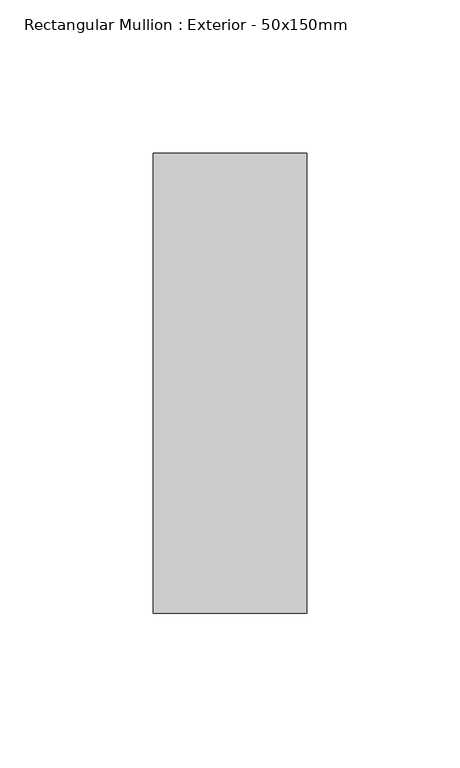
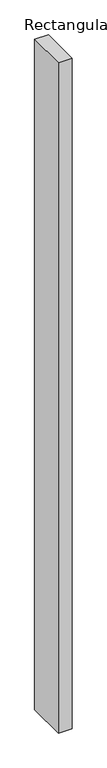
"""IFC4 building model written with IfcOpenShell, lengths in millimetres: member geometry, Rectangular Mullion : Exterior - 50x150mm."""

from ifc_helpers import new_model, si_unit, frame, origin, place, context, project, spatial, polyline, outline, extrude, source, transform, mapped, element, save


def rectangular_mullion_exterior_50x150mm_be5f20bc(model_context):
    return source(origin(), model_context, "Body", "SweptSolid", [
        extrude(outline(polyline([(25.0, 0.0), (25.0, -150.0), (-25.0, -150.0), (-25.0, 0.0), (25.0, 0.0)])), frame((0.0, 0.0, -2600.0), z_axis=(0.0, 0.0, 1.0), x_axis=(1.0, 0.0, 0.0)), (0.0, 0.0, 1.0), 2600.0),
    ])


if __name__ == "__main__":
    model = new_model("IFC4")
    model_context = context("Model", 3, world=origin())
    ifc_project = project(units=[si_unit("LENGTHUNIT", "METRE", prefix="MILLI")], contexts=[model_context])
    site = spatial("IfcSite", under=ifc_project)
    building = spatial("IfcBuilding", under=site)
    placement = place(None, origin())
    rectangular_mullion_exterior_50x150mm_shape = rectangular_mullion_exterior_50x150mm_be5f20bc(model_context)
    element("IfcMember", 1, ObjectType="Rectangular Mullion : Exterior - 50x150mm", at=placement, inside=building, context=model_context, shape_type="MappedRepresentation", body=[
        mapped(rectangular_mullion_exterior_50x150mm_shape, transform((0.0, 0.0, 0.0), x_axis=(1.0, 0.0, 0.0), y_axis=(0.0, 1.0, 0.0), z_axis=(0.0, 0.0, 1.0))),
    ])
    save(model, "model.ifc")

# Revit data of these elements
# Type "Rectangular Mullion : Exterior - 50x150mm"
#   built-in parameter 1007351 = -0.246063 (stored number, unit not read)
#   built-in parameter 1007304 = 0.492126 (stored number, unit not read)
#   built-in parameter 1007301 = 0.082021 (stored number, unit not read)
#   built-in parameter 1007300 = 0.082021 (stored number, unit not read)
# Element 1 (IfcMember, "Rectangular Mullion : Exterior - 50x150mm")
#   Materials on its faces: "Default Frame/Mullion (Interior/Exterior)"
# Materials
#   "Default Frame/Mullion (Interior/Exterior)": class "Generic", colour RGB 205 205 205, transparency 0, Description = "Udefineret karm/ramme materiale", Cost = 0
